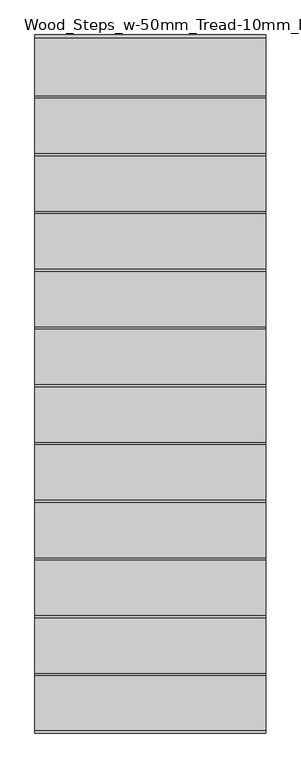
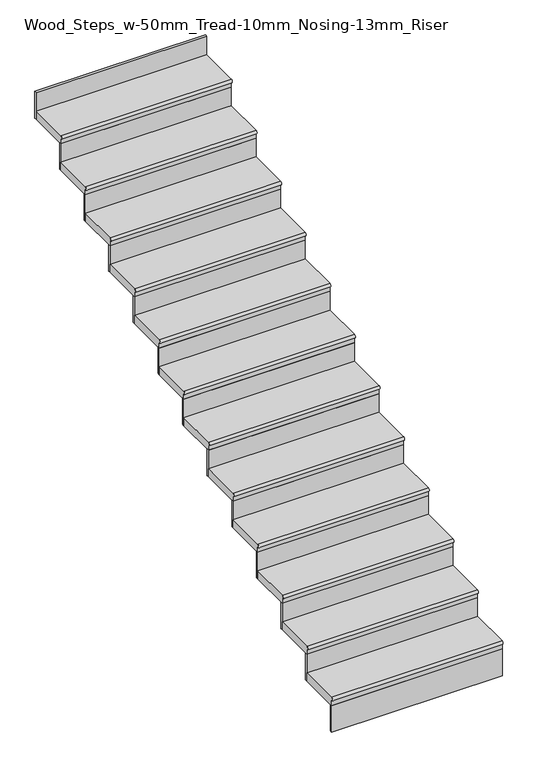
"""IFC4 building model written with IfcOpenShell, lengths in millimetres: stair flight geometry, Wood_Steps_w-50mm_Tread-10mm_Nosing-13mm_Riser."""

from ifc_helpers import new_model, si_unit, point, frame, frame_2d, origin, place, context, project, spatial, polyline, circle_curve, trimmed, segment, composite_curve, outline, extrude, source, transform, mapped, element, save


def wood_steps_w_50mm_tread_10mm_nosing_13mm_riser_78d7f248(model_context):
    return source(origin(), model_context, "Body", "SweptSolid", [
        extrude(outline(composite_curve([segment(polyline([(-2585.3813072, 823.5294118), (-2335.3813072, 823.5294118), (-2335.3813072, 773.5294118), (-2585.3813072, 773.5294118), (-2585.3813072, 803.5294118)]), True, "CONTINUOUS"), segment(trimmed(circle_curve(frame_2d((-2585.3813072, 813.5294118)), 10.0), [point((-2585.3813072, 803.5294118))], [point((-2585.3813072, 823.5294118))], False, "CARTESIAN"), True, "CONTINUOUS")], self_intersect=False)), frame((-3675.5365014, 0.0, 0.0), z_axis=(1.0, 0.0, 0.0), x_axis=(0.0, 1.0, 0.0)), (0.0, 0.0, 1.0), 1000.0),
        extrude(outline(polyline([(-2675.5365014, -2572.8813072), (-2675.5365014, -2585.3813072), (-3675.5365014, -2585.3813072), (-3675.5365014, -2572.8813072), (-2675.5365014, -2572.8813072)])), frame((0.0, 0.0, 608.8235294), z_axis=(0.0, 0.0, 1.0), x_axis=(1.0, 0.0, 0.0)), (0.0, 0.0, 1.0), 164.7058824),
        extrude(outline(polyline([(-2675.5365014, -2322.8813072), (-2675.5365014, -2335.3813072), (-3675.5365014, -2335.3813072), (-3675.5365014, -2322.8813072), (-2675.5365014, -2322.8813072)])), frame((0.0, 0.0, 773.5294118), z_axis=(0.0, 0.0, 1.0), x_axis=(1.0, 0.0, 0.0)), (0.0, 0.0, 1.0), 164.7058824),
        extrude(outline(composite_curve([segment(polyline([(-2335.3813072, 988.2352941), (-2085.3813072, 988.2352941), (-2085.3813072, 938.2352941), (-2335.3813072, 938.2352941), (-2335.3813072, 968.2352941)]), True, "CONTINUOUS"), segment(trimmed(circle_curve(frame_2d((-2335.3813072, 978.2352941)), 10.0), [point((-2335.3813072, 968.2352941))], [point((-2335.3813072, 988.2352941))], False, "CARTESIAN"), True, "CONTINUOUS")], self_intersect=False)), frame((-3675.5365014, 0.0, 0.0), z_axis=(1.0, 0.0, 0.0), x_axis=(0.0, 1.0, 0.0)), (0.0, 0.0, 1.0), 1000.0),
        extrude(outline(polyline([(-2675.5365014, -2072.8813072), (-2675.5365014, -2085.3813072), (-3675.5365014, -2085.3813072), (-3675.5365014, -2072.8813072), (-2675.5365014, -2072.8813072)])), frame((0.0, 0.0, 938.2352941), z_axis=(0.0, 0.0, 1.0), x_axis=(1.0, 0.0, 0.0)), (0.0, 0.0, 1.0), 164.7058824),
        extrude(outline(composite_curve([segment(polyline([(-2085.3813072, 1152.9411765), (-1835.3813072, 1152.9411765), (-1835.3813072, 1102.9411765), (-2085.3813072, 1102.9411765), (-2085.3813072, 1132.9411765)]), True, "CONTINUOUS"), segment(trimmed(circle_curve(frame_2d((-2085.3813072, 1142.9411765)), 10.0), [point((-2085.3813072, 1132.9411765))], [point((-2085.3813072, 1152.9411765))], False, "CARTESIAN"), True, "CONTINUOUS")], self_intersect=False)), frame((-3675.5365014, 0.0, 0.0), z_axis=(1.0, 0.0, 0.0), x_axis=(0.0, 1.0, 0.0)), (0.0, 0.0, 1.0), 1000.0),
        extrude(outline(polyline([(-2675.5365014, -1822.8813072), (-2675.5365014, -1835.3813072), (-3675.5365014, -1835.3813072), (-3675.5365014, -1822.8813072), (-2675.5365014, -1822.8813072)])), frame((0.0, 0.0, 1102.9411765), z_axis=(0.0, 0.0, 1.0), x_axis=(1.0, 0.0, 0.0)), (0.0, 0.0, 1.0), 164.7058824),
        extrude(outline(composite_curve([segment(polyline([(-1835.3813072, 1317.6470588), (-1585.3813072, 1317.6470588), (-1585.3813072, 1267.6470588), (-1835.3813072, 1267.6470588), (-1835.3813072, 1297.6470588)]), True, "CONTINUOUS"), segment(trimmed(circle_curve(frame_2d((-1835.3813072, 1307.6470588)), 10.0), [point((-1835.3813072, 1297.6470588))], [point((-1835.3813072, 1317.6470588))], False, "CARTESIAN"), True, "CONTINUOUS")], self_intersect=False)), frame((-3675.5365014, 0.0, 0.0), z_axis=(1.0, 0.0, 0.0), x_axis=(0.0, 1.0, 0.0)), (0.0, 0.0, 1.0), 1000.0),
        extrude(outline(polyline([(-2675.5365014, -1572.8813072), (-2675.5365014, -1585.3813072), (-3675.5365014, -1585.3813072), (-3675.5365014, -1572.8813072), (-2675.5365014, -1572.8813072)])), frame((0.0, 0.0, 1267.6470588), z_axis=(0.0, 0.0, 1.0), x_axis=(1.0, 0.0, 0.0)), (0.0, 0.0, 1.0), 164.7058824),
        extrude(outline(composite_curve([segment(polyline([(-1585.3813072, 1482.3529412), (-1335.3813072, 1482.3529412), (-1335.3813072, 1432.3529412), (-1585.3813072, 1432.3529412), (-1585.3813072, 1462.3529412)]), True, "CONTINUOUS"), segment(trimmed(circle_curve(frame_2d((-1585.3813072, 1472.3529412)), 10.0), [point((-1585.3813072, 1462.3529412))], [point((-1585.3813072, 1482.3529412))], False, "CARTESIAN"), True, "CONTINUOUS")], self_intersect=False)), frame((-3675.5365014, 0.0, 0.0), z_axis=(1.0, 0.0, 0.0), x_axis=(0.0, 1.0, 0.0)), (0.0, 0.0, 1.0), 1000.0),
        extrude(outline(polyline([(-2675.5365014, -1322.8813072), (-2675.5365014, -1335.3813072), (-3675.5365014, -1335.3813072), (-3675.5365014, -1322.8813072), (-2675.5365014, -1322.8813072)])), frame((0.0, 0.0, 1432.3529412), z_axis=(0.0, 0.0, 1.0), x_axis=(1.0, 0.0, 0.0)), (0.0, 0.0, 1.0), 164.7058824),
        extrude(outline(composite_curve([segment(polyline([(-1335.3813072, 1647.0588235), (-1085.3813072, 1647.0588235), (-1085.3813072, 1597.0588235), (-1335.3813072, 1597.0588235), (-1335.3813072, 1627.0588235)]), True, "CONTINUOUS"), segment(trimmed(circle_curve(frame_2d((-1335.3813072, 1637.0588235)), 10.0), [point((-1335.3813072, 1627.0588235))], [point((-1335.3813072, 1647.0588235))], False, "CARTESIAN"), True, "CONTINUOUS")], self_intersect=False)), frame((-3675.5365014, 0.0, 0.0), z_axis=(1.0, 0.0, 0.0), x_axis=(0.0, 1.0, 0.0)), (0.0, 0.0, 1.0), 1000.0),
        extrude(outline(polyline([(-2675.5365014, -1072.8813072), (-2675.5365014, -1085.3813072), (-3675.5365014, -1085.3813072), (-3675.5365014, -1072.8813072), (-2675.5365014, -1072.8813072)])), frame((0.0, 0.0, 1597.0588235), z_axis=(0.0, 0.0, 1.0), x_axis=(1.0, 0.0, 0.0)), (0.0, 0.0, 1.0), 164.7058824),
        extrude(outline(composite_curve([segment(polyline([(-1085.3813072, 1811.7647059), (-835.3813072, 1811.7647059), (-835.3813072, 1761.7647059), (-1085.3813072, 1761.7647059), (-1085.3813072, 1791.7647059)]), True, "CONTINUOUS"), segment(trimmed(circle_curve(frame_2d((-1085.3813072, 1801.7647059)), 10.0), [point((-1085.3813072, 1791.7647059))], [point((-1085.3813072, 1811.7647059))], False, "CARTESIAN"), True, "CONTINUOUS")], self_intersect=False)), frame((-3675.5365014, 0.0, 0.0), z_axis=(1.0, 0.0, 0.0), x_axis=(0.0, 1.0, 0.0)), (0.0, 0.0, 1.0), 1000.0),
        extrude(outline(polyline([(-2675.5365014, -822.8813072), (-2675.5365014, -835.3813072), (-3675.5365014, -835.3813072), (-3675.5365014, -822.8813072), (-2675.5365014, -822.8813072)])), frame((0.0, 0.0, 1761.7647059), z_axis=(0.0, 0.0, 1.0), x_axis=(1.0, 0.0, 0.0)), (0.0, 0.0, 1.0), 164.7058824),
        extrude(outline(composite_curve([segment(polyline([(-835.3813072, 1976.4705882), (-585.3813072, 1976.4705882), (-585.3813072, 1926.4705882), (-835.3813072, 1926.4705882), (-835.3813072, 1956.4705882)]), True, "CONTINUOUS"), segment(trimmed(circle_curve(frame_2d((-835.3813072, 1966.4705882)), 10.0), [point((-835.3813072, 1956.4705882))], [point((-835.3813072, 1976.4705882))], False, "CARTESIAN"), True, "CONTINUOUS")], self_intersect=False)), frame((-3675.5365014, 0.0, 0.0), z_axis=(1.0, 0.0, 0.0), x_axis=(0.0, 1.0, 0.0)), (0.0, 0.0, 1.0), 1000.0),
        extrude(outline(polyline([(-2675.5365014, -572.8813072), (-2675.5365014, -585.3813072), (-3675.5365014, -585.3813072), (-3675.5365014, -572.8813072), (-2675.5365014, -572.8813072)])), frame((0.0, 0.0, 1926.4705882), z_axis=(0.0, 0.0, 1.0), x_axis=(1.0, 0.0, 0.0)), (0.0, 0.0, 1.0), 164.7058824),
        extrude(outline(composite_curve([segment(polyline([(-585.3813072, 2141.1764706), (-335.3813072, 2141.1764706), (-335.3813072, 2091.1764706), (-585.3813072, 2091.1764706), (-585.3813072, 2121.1764706)]), True, "CONTINUOUS"), segment(trimmed(circle_curve(frame_2d((-585.3813072, 2131.1764706)), 10.0), [point((-585.3813072, 2121.1764706))], [point((-585.3813072, 2141.1764706))], False, "CARTESIAN"), True, "CONTINUOUS")], self_intersect=False)), frame((-3675.5365014, 0.0, 0.0), z_axis=(1.0, 0.0, 0.0), x_axis=(0.0, 1.0, 0.0)), (0.0, 0.0, 1.0), 1000.0),
        extrude(outline(polyline([(-2675.5365014, -322.8813072), (-2675.5365014, -335.3813072), (-3675.5365014, -335.3813072), (-3675.5365014, -322.8813072), (-2675.5365014, -322.8813072)])), frame((0.0, 0.0, 2091.1764706), z_axis=(0.0, 0.0, 1.0), x_axis=(1.0, 0.0, 0.0)), (0.0, 0.0, 1.0), 164.7058824),
        extrude(outline(composite_curve([segment(polyline([(-335.3813072, 2305.8823529), (-85.3813072, 2305.8823529), (-85.3813072, 2255.8823529), (-335.3813072, 2255.8823529), (-335.3813072, 2285.8823529)]), True, "CONTINUOUS"), segment(trimmed(circle_curve(frame_2d((-335.3813072, 2295.8823529)), 10.0), [point((-335.3813072, 2285.8823529))], [point((-335.3813072, 2305.8823529))], False, "CARTESIAN"), True, "CONTINUOUS")], self_intersect=False)), frame((-3675.5365014, 0.0, 0.0), z_axis=(1.0, 0.0, 0.0), x_axis=(0.0, 1.0, 0.0)), (0.0, 0.0, 1.0), 1000.0),
        extrude(outline(polyline([(-2675.5365014, -72.8813072), (-2675.5365014, -85.3813072), (-3675.5365014, -85.3813072), (-3675.5365014, -72.8813072), (-2675.5365014, -72.8813072)])), frame((0.0, 0.0, 2255.8823529), z_axis=(0.0, 0.0, 1.0), x_axis=(1.0, 0.0, 0.0)), (0.0, 0.0, 1.0), 164.7058824),
        extrude(outline(composite_curve([segment(polyline([(-85.3813072, 2470.5882353), (164.6186928, 2470.5882353), (164.6186928, 2420.5882353), (-85.3813072, 2420.5882353), (-85.3813072, 2450.5882353)]), True, "CONTINUOUS"), segment(trimmed(circle_curve(frame_2d((-85.3813072, 2460.5882353)), 10.0), [point((-85.3813072, 2450.5882353))], [point((-85.3813072, 2470.5882353))], False, "CARTESIAN"), True, "CONTINUOUS")], self_intersect=False)), frame((-3675.5365014, 0.0, 0.0), z_axis=(1.0, 0.0, 0.0), x_axis=(0.0, 1.0, 0.0)), (0.0, 0.0, 1.0), 1000.0),
        extrude(outline(polyline([(-2675.5365014, 177.1186928), (-2675.5365014, 164.6186928), (-3675.5365014, 164.6186928), (-3675.5365014, 177.1186928), (-2675.5365014, 177.1186928)])), frame((0.0, 0.0, 2420.5882353), z_axis=(0.0, 0.0, 1.0), x_axis=(1.0, 0.0, 0.0)), (0.0, 0.0, 1.0), 164.7058824),
        extrude(outline(polyline([(-2675.5365014, 427.1186928), (-2675.5365014, 414.6186928), (-3675.5365014, 414.6186928), (-3675.5365014, 427.1186928), (-2675.5365014, 427.1186928)])), frame((0.0, 0.0, 2585.2941176), z_axis=(0.0, 0.0, 1.0), x_axis=(1.0, 0.0, 0.0)), (0.0, 0.0, 1.0), 164.7058824),
        extrude(outline(composite_curve([segment(polyline([(164.6186928, 2635.2941176), (414.6186928, 2635.2941176), (414.6186928, 2585.2941176), (164.6186928, 2585.2941176), (164.6186928, 2615.2941176)]), True, "CONTINUOUS"), segment(trimmed(circle_curve(frame_2d((164.6186928, 2625.2941176)), 10.0), [point((164.6186928, 2615.2941176))], [point((164.6186928, 2635.2941176))], False, "CARTESIAN"), True, "CONTINUOUS")], self_intersect=False)), frame((-3675.5365014, 0.0, 0.0), z_axis=(1.0, 0.0, 0.0), x_axis=(0.0, 1.0, 0.0)), (0.0, 0.0, 1.0), 1000.0),
    ])


if __name__ == "__main__":
    model = new_model("IFC4")
    model_context = context("Model", 3, world=origin())
    ifc_project = project(units=[si_unit("LENGTHUNIT", "METRE", prefix="MILLI")], contexts=[model_context])
    site = spatial("IfcSite", under=ifc_project)
    building = spatial("IfcBuilding", under=site)
    placement = place(None, origin())
    wood_steps_w_50mm_tread_10mm_nosing_13mm_riser_shape = wood_steps_w_50mm_tread_10mm_nosing_13mm_riser_78d7f248(model_context)
    element("IfcStairFlight", 1, ObjectType="Wood_Steps_w-50mm_Tread-10mm_Nosing-13mm_Riser", at=placement, inside=building, context=model_context, shape_type="MappedRepresentation", body=[
        mapped(wood_steps_w_50mm_tread_10mm_nosing_13mm_riser_shape, transform((0.0, 0.0, 0.0), x_axis=(1.0, 0.0, 0.0), y_axis=(0.0, 1.0, 0.0), z_axis=(0.0, 0.0, 1.0))),
    ])
    save(model, "model.ifc")

# Revit data of these elements
# Element 1 (IfcStairFlight, "Wood_Steps_w-50mm_Tread-10mm_Nosing-13mm_Riser")
#   Materials on its faces: "Oak Flooring"
# Materials
#   "Oak Flooring": class "Wood", colour RGB 212 179 113, transparency 0, Description = "Quercus Rubra", Cost = 0
